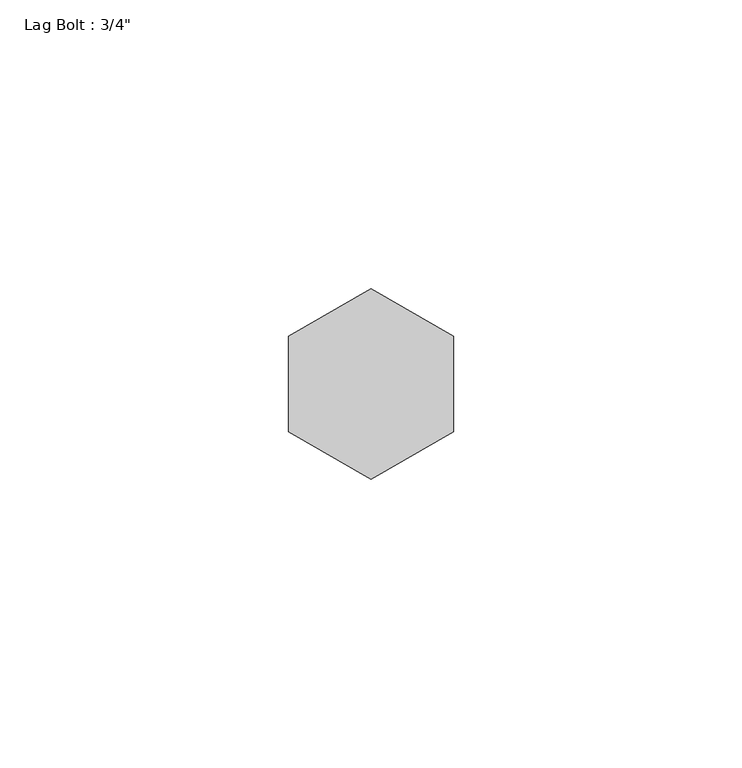
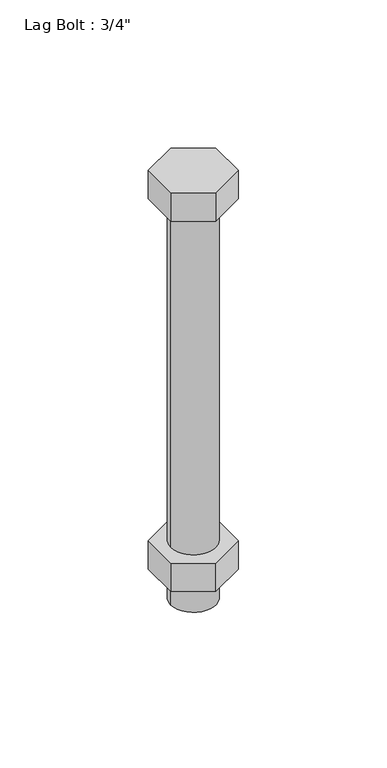
"""IFC4 building model written with IfcOpenShell, lengths in millimetres: proxy geometry."""

from ifc_helpers import new_model, si_unit, point, frame, origin, origin_with_axes, origin_2d, place, context, project, spatial, polyline, circle_curve, trimmed, segment, composite_curve, outline, extrude, source, transform, mapped, element, save


def proxy_a8761b9c(model_context):
    return source(origin(), model_context, "Body", "SweptSolid", [
        extrude(outline(polyline([(-14.2875, -8.248892), (-14.2875, 8.248892), (0.0, 16.4977839), (14.2875, 8.248892), (14.2875, -8.248892), (0.0, -16.4977839), (-14.2875, -8.248892)])), frame((0.0, 0.0, -165.1), z_axis=(0.0, 0.0, 1.0), x_axis=(1.0, 0.0, 0.0)), (0.0, 0.0, 1.0), 12.7),
        extrude(outline(polyline([(-14.2875, 8.248892), (0.0, 16.4977839), (14.2875, 8.248892), (14.2875, -8.248892), (0.0, -16.4977839), (-14.2875, -8.248892), (-14.2875, 8.248892)])), origin_with_axes(), (0.0, 0.0, 1.0), 12.7),
        extrude(outline(composite_curve([segment(trimmed(circle_curve(origin_2d(), 9.525), [point((-9.525, 0.0))], [point((9.525, 0.0))], False, "CARTESIAN"), True, "CONTINUOUS"), segment(trimmed(circle_curve(origin_2d(), 9.525), [point((9.525, 0.0))], [point((-9.525, 0.0))], False, "CARTESIAN"), True, "CONTINUOUS")], self_intersect=False)), frame((0.0, 0.0, -177.8), z_axis=(0.0, 0.0, 1.0), x_axis=(1.0, 0.0, 0.0)), (0.0, 0.0, 1.0), 177.8),
    ])


if __name__ == "__main__":
    model = new_model("IFC4")
    model_context = context("Model", 3, world=origin())
    ifc_project = project(units=[si_unit("LENGTHUNIT", "METRE", prefix="MILLI")], contexts=[model_context])
    site = spatial("IfcSite", under=ifc_project)
    building = spatial("IfcBuilding", under=site)
    placement = place(None, origin())
    proxy_shape = proxy_a8761b9c(model_context)
    element("IfcBuildingElementProxy", 1, Name="Lag Bolt : 3/4\"", ObjectType="Lag Bolt : 3/4\"", at=placement, inside=building, context=model_context, shape_type="MappedRepresentation", body=[
        mapped(proxy_shape, transform((0.0, 0.0, 0.0), x_axis=(1.0, 0.0, 0.0), y_axis=(0.0, 1.0, 0.0), z_axis=(0.0, 0.0, 1.0))),
    ])
    save(model, "model.ifc")

# Revit data of these elements
# Type "Lag Bolt : 3/4\""
#   Thickness_of_Substrate [instance default] = 0' - 1"
#   Side = 0' - 0.65039"
#   Radius = 0' - 0 3/8"
#   Length = 0' - 7"
#   Head Size = 0' - 1 1/8"
#   Head Radius = 0' - 0 9/16"
#   Head Height = 0' - 0 1/2"
#   Diameter = 0' - 0 3/4"
#   Default Elevation = 4' - 0"
#   Nut_Visibility [instance default] = yes
#   Bolt Material (Size) [instance default] = 5/8" GALV. ANCHOR BOLT @ 24" O.C. (6" MIN. EMBEDMENT)
# Element 1 (IfcBuildingElementProxy, "Lag Bolt : 3/4\"")
#   Thickness_of_Substrate = 0' - 6"
#   Bolt Material (Size) = 3/4" THU BOLT (RAW STEEL)
#   Materials on its faces: "3/4\" THU BOLT (RAW STEEL)"
# Materials
#   "5/8\" GALV. ANCHOR BOLT @ 24\" O.C. (6\" MIN. EMBEDMENT)": class "Generic", colour RGB 120 120 120, transparency 0, Cost = 0
#   "3/4\" THU BOLT (RAW STEEL)": class "Generic", colour RGB 120 120 120, transparency 0, Cost = 0
